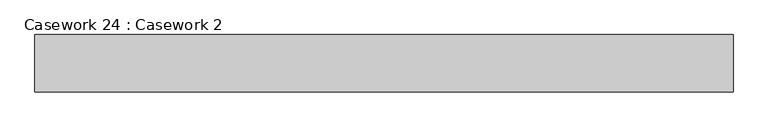
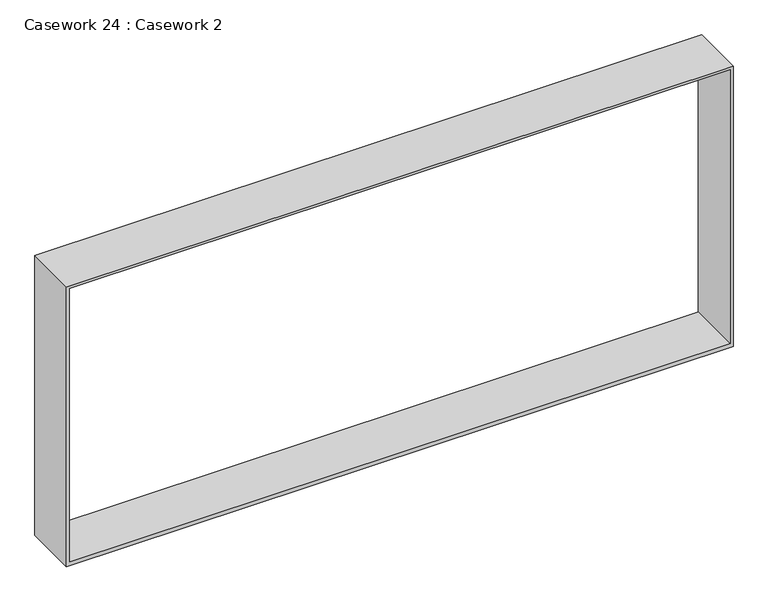
"""IFC4 building model written with IfcOpenShell, lengths in millimetres: furniture geometry, Casework 24 : Casework 2."""

import ifcopenshell
import ifcopenshell.guid

model = None  # the IFC model being written
_history = None  # IfcOwnerHistory: only IFC2X3 demands one
_inside = {}  # id of a spatial element -> (the spatial element, [elements in it])
_under = {}  # id of a project, library or spatial element -> (it, [spatial elements below it])
_declared = {}  # id of a project -> (the project, [libraries it declares])
_typed = {}  # id of a type object -> (the type object, [elements of that type])
_made_of = {}  # id of a material, layer set ... -> (it, [elements and type objects made of it])


def new_model(schema):
    """Start an empty IFC model of exactly this schema.

    Asked for "IFC4X3", IfcOpenShell would pick the latest addendum, in which some entities
    have other attributes; the version numbers below select the first issue.
    IFC2X3 requires an IfcOwnerHistory on every rooted entity: one is made here for all.
    """
    global model, _history
    if schema == "IFC4X3":
        model = ifcopenshell.file(schema_version=(4, 3, 0, 0))
    else:
        model = ifcopenshell.file(schema=schema)
    _inside.clear()
    _under.clear()
    _declared.clear()
    _typed.clear()
    _made_of.clear()
    _history = None
    if model.schema == "IFC2X3":
        org = make("IfcOrganization", Name="unknown")
        user = make(
            "IfcPersonAndOrganization",
            ThePerson=make("IfcPerson", FamilyName="unknown"),
            TheOrganization=org,
        )
        app = make(
            "IfcApplication",
            ApplicationDeveloper=org,
            Version="unknown",
            ApplicationFullName="unknown",
            ApplicationIdentifier="unknown",
        )
        _history = make(
            "IfcOwnerHistory",
            OwningUser=user,
            OwningApplication=app,
            ChangeAction="ADDED",
            CreationDate=0,
        )
    return model


def make(cls, **values):
    """One entity of the class cls with the attributes given. An attribute that is None is left unset."""
    return model.create_entity(
        cls, **{name: value for name, value in values.items() if value is not None}
    )


def rooted(cls, **values):
    """An entity with a GlobalId (a new one), such as an element, a storey or a relation."""
    return make(cls, GlobalId=ifcopenshell.guid.new(), OwnerHistory=_history, **values)


def si_unit(unit_type, name, prefix=None):
    """IfcSIUnit, for example si_unit("LENGTHUNIT", "METRE", prefix="MILLI")."""
    return make("IfcSIUnit", UnitType=unit_type, Prefix=prefix, Name=name)


def assignment(units):
    """IfcUnitAssignment: the units of a project."""
    return None if units is None else make("IfcUnitAssignment", Units=units)


def point(xyz):
    """IfcCartesianPoint."""
    return None if xyz is None else make("IfcCartesianPoint", Coordinates=xyz)


def direction(xyz):
    """IfcDirection."""
    return None if xyz is None else make("IfcDirection", DirectionRatios=xyz)


def frame(location, z_axis=None, x_axis=None):
    """IfcAxis2Placement3D, a coordinate frame: its origin and axes. An axis left out is left unset."""
    return make(
        "IfcAxis2Placement3D",
        Location=point(location),
        Axis=direction(z_axis),
        RefDirection=direction(x_axis),
    )


def origin():
    """The frame at (0, 0, 0) with its axes left unset."""
    return frame((0.0, 0.0, 0.0))


def place(relative_to, where):
    """IfcLocalPlacement: puts the frame where relative to a parent placement (None: the world)."""
    return make(
        "IfcLocalPlacement", PlacementRelTo=relative_to, RelativePlacement=where
    )


def context(
    kind, dimensions, precision=None, world=None, true_north=None, identifier=None
):
    """IfcGeometricRepresentationContext, for example the 3D "Model" context."""
    return make(
        "IfcGeometricRepresentationContext",
        ContextIdentifier=identifier,
        ContextType=kind,
        CoordinateSpaceDimension=dimensions,
        Precision=precision,
        WorldCoordinateSystem=world,
        TrueNorth=true_north,
    )


def project(units=None, contexts=None):
    """IfcProject with its units and contexts."""
    return rooted(
        "IfcProject",
        Name="project",
        RepresentationContexts=contexts,
        UnitsInContext=assignment(units),
    )


def spatial(cls, under=None, at=None, **own):
    """A site, building, storey or space (cls), placed at a placement, below another one or the project."""
    s = rooted(cls, ObjectPlacement=at, **own)
    if under is not None:
        _under.setdefault(under.id(), (under, []))[1].append(s)
    return s


def polyline(points):
    """IfcPolyline through the points."""
    return make("IfcPolyline", Points=[point(p) for p in points])


def outline(outer, holes=None, kind="AREA"):
    """IfcArbitraryClosedProfileDef: a profile drawn as a closed curve; with holes, ...WithVoids."""
    if holes is None:
        return make("IfcArbitraryClosedProfileDef", ProfileType=kind, OuterCurve=outer)
    return make(
        "IfcArbitraryProfileDefWithVoids",
        ProfileType=kind,
        OuterCurve=outer,
        InnerCurves=holes,
    )


def extrude(swept, where, along, depth):
    """IfcExtrudedAreaSolid: the profile swept, set in the frame where, extruded along a direction by depth."""
    return make(
        "IfcExtrudedAreaSolid",
        SweptArea=swept,
        Position=where,
        ExtrudedDirection=direction(along),
        Depth=depth,
    )


def shape(context_of_items, identifier, shape_type, items):
    """IfcShapeRepresentation: the items that make up one representation, for example the "Body"."""
    return make(
        "IfcShapeRepresentation",
        ContextOfItems=context_of_items,
        RepresentationIdentifier=identifier,
        RepresentationType=shape_type,
        Items=items,
    )


def source(mapping_origin, context_of_items, identifier, shape_type, items):
    """IfcRepresentationMap: a shape defined once, which mapped items show again and again."""
    return make(
        "IfcRepresentationMap",
        MappingOrigin=mapping_origin,
        MappedRepresentation=shape(context_of_items, identifier, shape_type, items),
    )


def transform(
    local_origin,
    x_axis=None,
    y_axis=None,
    z_axis=None,
    scale=None,
    scale2=None,
    scale3=None,
    uniform=True,
):
    """IfcCartesianTransformationOperator3D, or its non-uniform kind. x_axis, y_axis, z_axis: its Axis1, 2, 3."""
    if uniform:
        return make(
            "IfcCartesianTransformationOperator3D",
            Axis1=direction(x_axis),
            Axis2=direction(y_axis),
            LocalOrigin=point(local_origin),
            Scale=scale,
            Axis3=direction(z_axis),
        )
    return make(
        "IfcCartesianTransformationOperator3DnonUniform",
        Axis1=direction(x_axis),
        Axis2=direction(y_axis),
        LocalOrigin=point(local_origin),
        Scale=scale,
        Axis3=direction(z_axis),
        Scale2=scale2,
        Scale3=scale3,
    )


def mapped(mapping_source, mapping_target):
    """IfcMappedItem: shows the shape of a source again, moved by a transform."""
    return make(
        "IfcMappedItem", MappingSource=mapping_source, MappingTarget=mapping_target
    )


def made_of(thing, what):
    """Note that an element or type object is made of a material, layer set ...; save() writes the relation."""
    if what is not None:
        _made_of.setdefault(what.id(), (what, []))[1].append(thing)
    return thing


def element(
    cls,
    number,
    at=None,
    inside=None,
    cuts=None,
    type_object=None,
    material=None,
    context=None,
    identifier="Body",
    shape_type=None,
    held_by="IfcProductDefinitionShape",
    body=None,
    shapes=None,
    **own,
):
    """One element of the class cls, such as IfcWall. Its Tag is "e" and its number.

    at: its placement. inside: the storey or other place that contains it. cuts: it is an
    opening in that element (IfcRelVoidsElement). A single representation is given by context,
    identifier, shape_type and body (its items); several are given by shapes. held_by: the class
    of the entity that holds the representations. save() writes the other relations.
    """
    e = rooted(cls, Tag="e%d" % number, ObjectPlacement=at, **own)
    if body is not None:
        shapes = [shape(context, identifier, shape_type, body)]
    if shapes is not None:
        e.Representation = make(held_by, Representations=shapes)
    if inside is not None:
        _inside.setdefault(inside.id(), (inside, []))[1].append(e)
    if cuts is not None:
        rooted(
            "IfcRelVoidsElement", RelatingBuildingElement=cuts, RelatedOpeningElement=e
        )
    if type_object is not None:
        _typed.setdefault(type_object.id(), (type_object, []))[1].append(e)
    return made_of(e, material)


def aggregate(whole, parts):
    """IfcRelAggregates: a whole, such as a stair, and the parts it consists of."""
    return rooted("IfcRelAggregates", RelatingObject=whole, RelatedObjects=parts)


def save(model, path):
    """Write the relations noted so far, then the file.

    IfcRelAggregates (storeys below a building ...), IfcRelContainedInSpatialStructure (elements
    in a storey), IfcRelDefinesByType, IfcRelAssociatesMaterial and IfcRelDeclares: one each for
    every whole, place, type object, material and project.
    """
    for whole, parts in _under.values():
        aggregate(whole, parts)
    for where, things in _inside.values():
        rooted(
            "IfcRelContainedInSpatialStructure",
            RelatedElements=things,
            RelatingStructure=where,
        )
    for kind, things in _typed.values():
        rooted("IfcRelDefinesByType", RelatedObjects=things, RelatingType=kind)
    for what, things in _made_of.values():
        rooted("IfcRelAssociatesMaterial", RelatedObjects=things, RelatingMaterial=what)
    for by, libraries in _declared.values():
        rooted("IfcRelDeclares", RelatingContext=by, RelatedDefinitions=libraries)
    model.write(path)


def casework_24_casework_2_4cfab9a8(model_context):
    return source(origin(), model_context, "Body", "SweptSolid", [
        extrude(outline(polyline([(3048.0, -58223.6551606), (609.6, -58223.6551606), (609.6, -52737.2551606), (3048.0, -52737.2551606), (3048.0, -58223.6551606)]), holes=[polyline([(3024.850107, -58198.2551606), (3024.850107, -52762.6551606), (643.13302, -52762.6551606), (643.13302, -58198.2551606), (3024.850107, -58198.2551606)])]), frame((0.0, 285614.3720148, 0.0), z_axis=(0.0, 1.0, 0.0), x_axis=(0.0, 0.0, 1.0)), (0.0, 0.0, 1.0), 450.1962661),
    ])


if __name__ == "__main__":
    model = new_model("IFC4")
    model_context = context("Model", 3, world=origin())
    ifc_project = project(units=[si_unit("LENGTHUNIT", "METRE", prefix="MILLI")], contexts=[model_context])
    site = spatial("IfcSite", under=ifc_project)
    building = spatial("IfcBuilding", under=site)
    placement = place(None, origin())
    casework_24_casework_2_shape = casework_24_casework_2_4cfab9a8(model_context)
    element("IfcFurniture", 1, ObjectType="Casework 24 : Casework 2", at=placement, inside=building, context=model_context, shape_type="MappedRepresentation", body=[
        mapped(casework_24_casework_2_shape, transform((0.0, 0.0, 0.0), x_axis=(1.0, 0.0, 0.0), y_axis=(0.0, 1.0, 0.0), z_axis=(0.0, 0.0, 1.0))),
    ])
    save(model, "model.ifc")

# Revit data of these elements
# Element 1 (IfcFurniture, "Casework 24 : Casework 2")
#   Materials on its faces: "Dark metal"
# Materials
#   "Dark metal": class "Generic", colour RGB 44 29 29, transparency 0, Cost = 0
